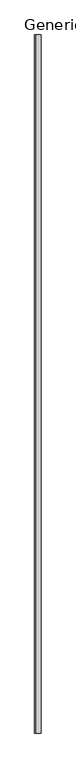
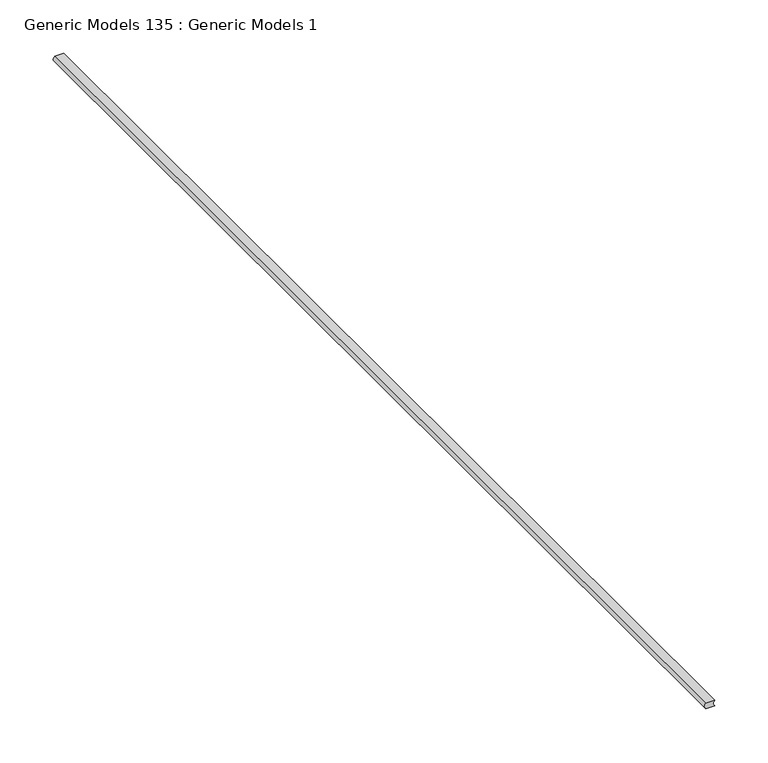
"""IFC4 building model written with IfcOpenShell, lengths in millimetres: proxy geometry, Generic Models 135 : Generic Models 1."""

from ifc_helpers import new_model, si_unit, point, frame, frame_2d, origin, place, context, project, spatial, polyline, circle_curve, trimmed, segment, composite_curve, outline, extrude, source, transform, mapped, element, save


def generic_models_135_generic_models_1_f2b08089(model_context):
    return source(origin(), model_context, "Body", "SweptSolid", [
        extrude(outline(composite_curve([segment(trimmed(circle_curve(frame_2d((-222.801067, 48169.1006666)), 4.3100275), [point((-225.976067, 48166.1859261))], [point((-219.626067, 48166.1859261))], True, "CARTESIAN"), True, "CONTINUOUS"), segment(polyline([(-219.626067, 48166.1859261), (-219.626067, 48156.6609261)]), True, "CONTINUOUS"), segment(trimmed(circle_curve(frame_2d((-222.801067, 48159.5756666)), 4.3100275), [point((-219.626067, 48156.6609261))], [point((-225.976067, 48156.6609261))], False, "CARTESIAN"), True, "CONTINUOUS"), segment(polyline([(-225.976067, 48156.6609261), (-225.976067, 48166.1859261)]), True, "CONTINUOUS")], self_intersect=False)), frame((0.0, 0.0, 0.0), z_axis=(0.0, 1.0, 0.0), x_axis=(0.0, 0.0, 1.0)), (0.0, 0.0, 1.0), 1219.2),
    ])


if __name__ == "__main__":
    model = new_model("IFC4")
    model_context = context("Model", 3, world=origin())
    ifc_project = project(units=[si_unit("LENGTHUNIT", "METRE", prefix="MILLI")], contexts=[model_context])
    site = spatial("IfcSite", under=ifc_project)
    building = spatial("IfcBuilding", under=site)
    placement = place(None, origin())
    generic_models_135_generic_models_1_shape = generic_models_135_generic_models_1_f2b08089(model_context)
    element("IfcBuildingElementProxy", 1, Name="Generic Models 135 : Generic Models 1", ObjectType="Generic Models 135 : Generic Models 1", at=placement, inside=building, context=model_context, shape_type="MappedRepresentation", body=[
        mapped(generic_models_135_generic_models_1_shape, transform((0.0, 0.0, 0.0), x_axis=(1.0, 0.0, 0.0), y_axis=(0.0, 1.0, 0.0), z_axis=(0.0, 0.0, 1.0))),
    ])
    save(model, "model.ifc")

# Revit data of these elements
# Element 1 (IfcBuildingElementProxy, "Generic Models 135 : Generic Models 1")
#   Materials on its faces: "SEALANT (W/ BACKER ROD IF NECESSARY)"
# Materials
#   "SEALANT (W/ BACKER ROD IF NECESSARY)": class "Unassigned", colour RGB 120 120 120, transparency 0, Cost = 0
